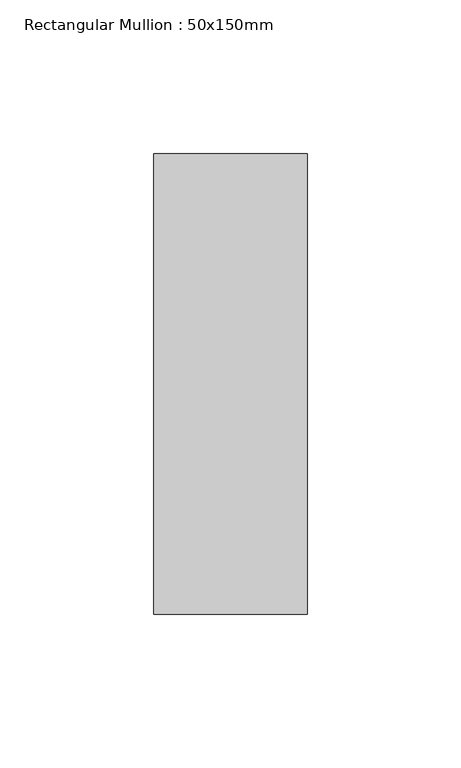
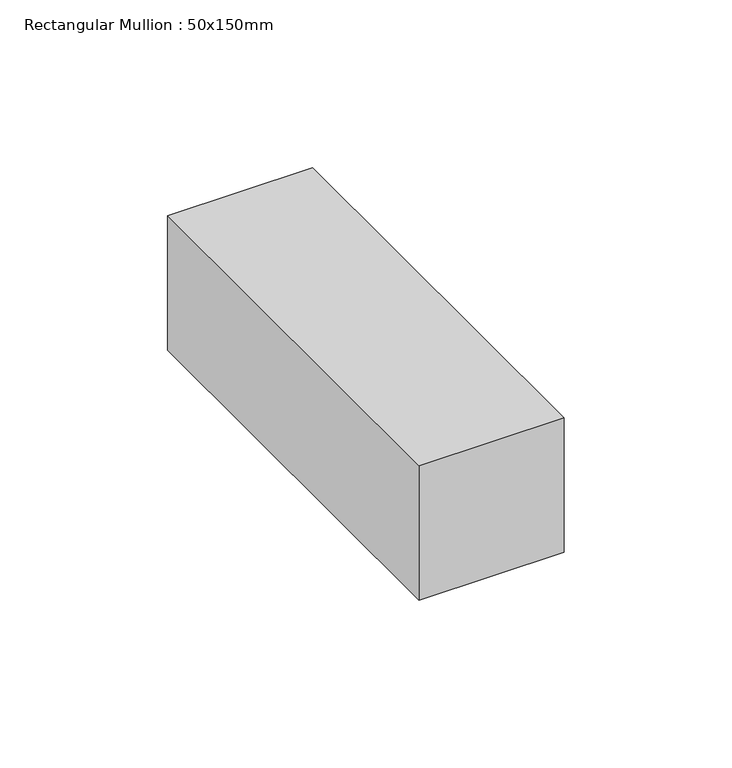
"""IFC4 building model written with IfcOpenShell, lengths in millimetres: member geometry, Rectangular Mullion : 50x150mm."""

from ifc_helpers import new_model, si_unit, frame, origin, place, context, project, spatial, polyline, outline, extrude, source, transform, mapped, element, save


def rectangular_mullion_50x150mm_9c05e6f5(model_context):
    return source(origin(), model_context, "Body", "SweptSolid", [
        extrude(outline(polyline([(0.0, 75.0), (0.0, -75.0), (-50.0, -75.0), (-50.0, 75.0), (0.0, 75.0)])), frame((0.0, 0.0, -49.0185145), z_axis=(0.0, 0.0, 1.0), x_axis=(1.0, 0.0, 0.0)), (0.0, 0.0, 1.0), 49.0185145),
    ])


if __name__ == "__main__":
    model = new_model("IFC4")
    model_context = context("Model", 3, world=origin())
    ifc_project = project(units=[si_unit("LENGTHUNIT", "METRE", prefix="MILLI")], contexts=[model_context])
    site = spatial("IfcSite", under=ifc_project)
    building = spatial("IfcBuilding", under=site)
    placement = place(None, origin())
    rectangular_mullion_50x150mm_shape = rectangular_mullion_50x150mm_9c05e6f5(model_context)
    element("IfcMember", 1, ObjectType="Rectangular Mullion : 50x150mm", at=placement, inside=building, context=model_context, shape_type="MappedRepresentation", body=[
        mapped(rectangular_mullion_50x150mm_shape, transform((0.0, 0.0, 0.0), x_axis=(1.0, 0.0, 0.0), y_axis=(0.0, 1.0, 0.0), z_axis=(0.0, 0.0, 1.0))),
    ])
    save(model, "model.ifc")

# Revit data of these elements
# Type "Rectangular Mullion : 50x150mm"
#   Keynote = "H11"
#   built-in parameter 1007304 = 0.492126 (stored number, unit not read)
#   built-in parameter 1007301 = 0.082021 (stored number, unit not read)
#   built-in parameter 1007300 = 0.082021 (stored number, unit not read)
# Element 1 (IfcMember, "Rectangular Mullion : 50x150mm")
#   Materials on its faces: "Aluminium"
# Materials
#   "Aluminium": class "Metal", colour RGB 247 247 247, transparency 0, Description = "Aluminium 6061", Cost = 0
